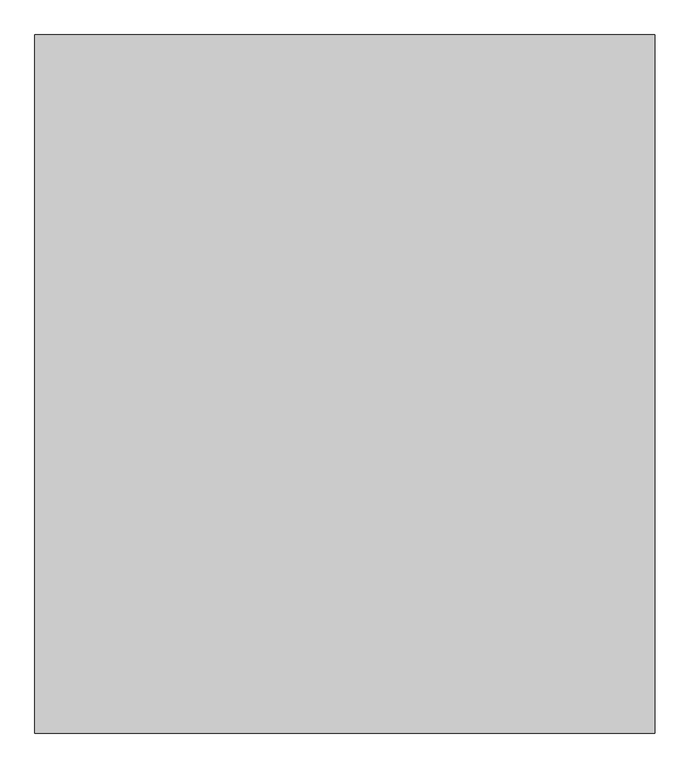
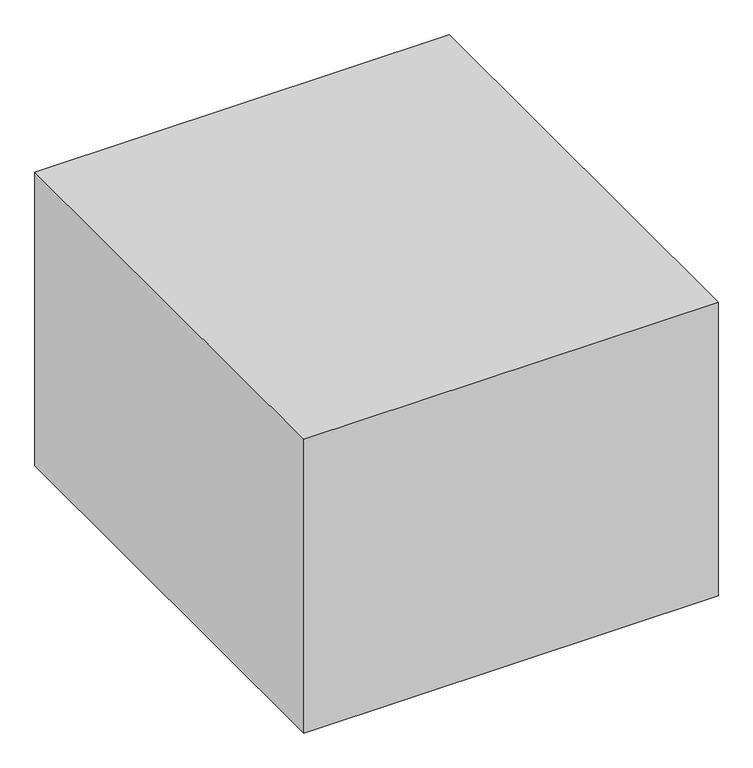
"""IFC4 building model written with IfcOpenShell, lengths in millimetres: proxy geometry, Space Planning Box_hec : Space Planning Box_hec."""

from ifc_helpers import new_model, si_unit, origin, origin_with_axes, place, context, project, spatial, polyline, outline, extrude, source, transform, mapped, element, save


def generic_models_4d084078(model_context):
    return source(origin(), model_context, "Body", "SweptSolid", [
        extrude(outline(polyline([(4000.0, 4500.0), (4000.0, -4500.0), (-4000.0, -4500.0), (-4000.0, 4500.0), (4000.0, 4500.0)])), origin_with_axes(), (0.0, 0.0, 1.0), 6000.0),
    ])


if __name__ == "__main__":
    model = new_model("IFC4")
    model_context = context("Model", 3, world=origin())
    ifc_project = project(units=[si_unit("LENGTHUNIT", "METRE", prefix="MILLI")], contexts=[model_context])
    site = spatial("IfcSite", under=ifc_project)
    building = spatial("IfcBuilding", under=site)
    placement = place(None, origin())
    generic_models_shape = generic_models_4d084078(model_context)
    element("IfcBuildingElementProxy", 1, Name="Space Planning Box_hec : Space Planning Box_hec", ObjectType="Space Planning Box_hec : Space Planning Box_hec", at=placement, inside=building, context=model_context, shape_type="MappedRepresentation", body=[
        mapped(generic_models_shape, transform((0.0, 0.0, 0.0), x_axis=(1.0, 0.0, 0.0), y_axis=(0.0, 1.0, 0.0), z_axis=(0.0, 0.0, 1.0))),
    ])
    save(model, "model.ifc")

# Revit data of these elements
# Type "Space Planning Box_hec : Space Planning Box_hec"
#   Type Comments = "..."
#   Room Name [instance default] = "?"
#   Interior Finish [instance default] = ""
#   Exterior Finish [instance default] = ""
#   Department [instance default] = ""
#   Assembly Code = "..."
#   Width [instance default] = 1524 mm
#   Program Area [instance default] = 0 m²
#   Length [instance default] = 1524 mm
#   Height [instance default] = 1524 mm
#   Area [instance default] = 2.32258 m²
#   Fill Color [instance default] = Cyan
#   Default Elevation = 0
# Element 1 (IfcBuildingElementProxy, "Space Planning Box_hec : Space Planning Box_hec")
#   Room Name = "Fire Gas Room"
#   Interior Finish = "IF1"
#   Exterior Finish = "EF1"
#   Department = "SF"
#   Width = 8000 mm
#   Length = 9000 mm
#   Height = 6000 mm
#   Area = 72 m²
#   Materials on its faces: "Cyan"
# Materials
#   "Cyan": class "Generic", colour RGB 0 255 255, transparency 0.2, Cost = 0
